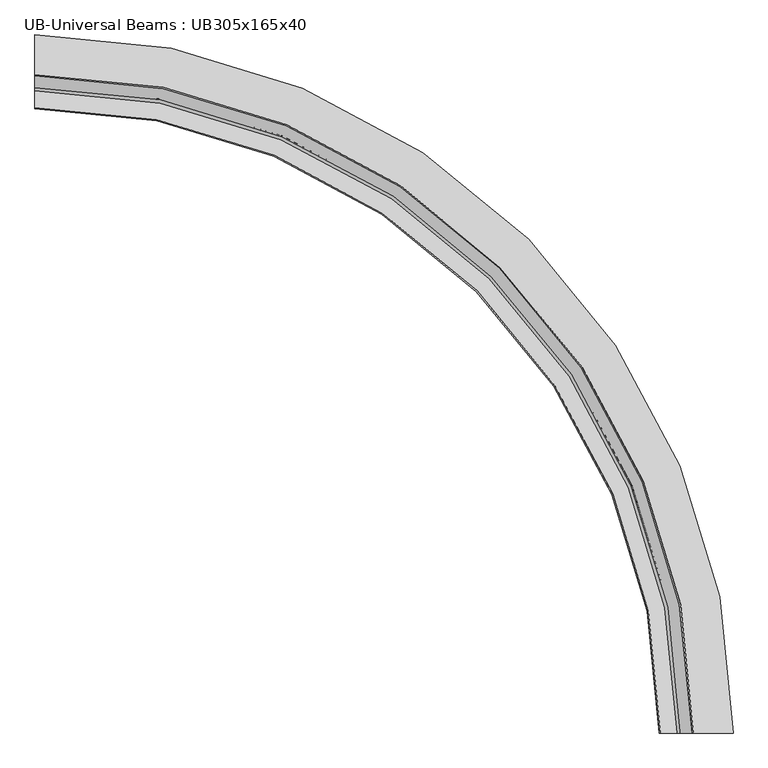
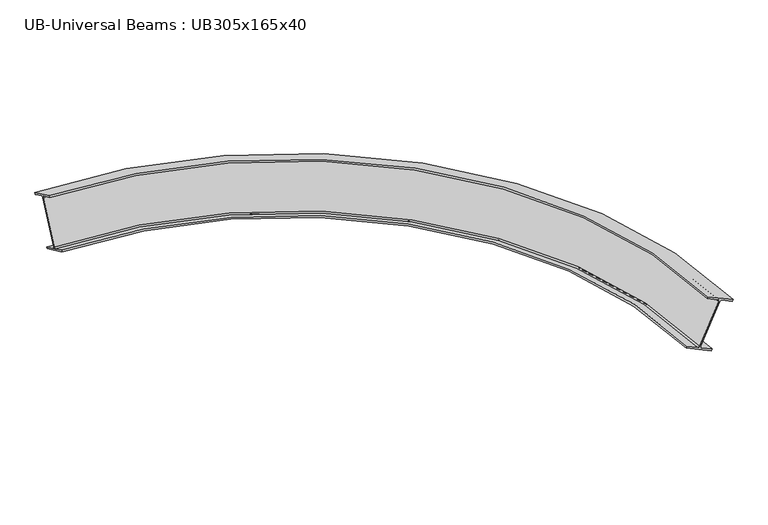
"""IFC4 building model written with IfcOpenShell, lengths in millimetres: beam geometry, UB-Universal Beams : UB305x165x40."""

from ifc_helpers import new_model, si_unit, point, frame, origin, place, context, project, spatial, polyline, circle_curve, ellipse_curve, trimmed, source, transform, mapped, element, save
from ifc_brep_helpers import plane_surface, revolved_surface, advanced_brep


def ub_universal_beams_ub305x165x40_80cf76f0(model_context):
    return source(origin(), model_context, "Body", "AdvancedBrep", [
        advanced_brep(
        [(2496.4431304, -2481.473222, -163.1085585), (2432.4578006, -2481.473222, -133.2717092), (2428.1529638, -2481.473222, -121.4442673), (2540.2313268, -2481.473222, 118.9085578), (2552.0587687, -2481.473222, 123.2133946), (2616.0440984, -2481.473222, 93.3765453), (2620.3548047, -2481.473222, 102.6208847), (2470.8140198, -2481.473222, 172.3528979), (2466.5033136, -2481.473222, 163.1085585), (2530.4886433, -2481.473222, 133.2717092), (2534.7934801, -2481.473222, 121.4442673), (2422.7151171, -2481.473222, -118.9085578), (2410.8876753, -2481.473222, -123.2133946), (2346.9023455, -2481.473222, -93.3765453), (2342.5916392, -2481.473222, -102.6208847), (2492.1324241, -2481.473222, -172.3528979), (0.0, 14.9699084, -163.1085585), (0.0, 10.6592021, -172.3528979), (0.0, -138.8815827, -102.6208847), (0.0, -134.5708765, -93.3765453), (0.0, -70.5855467, -123.2133946), (0.0, -58.7581049, -118.9085578), (0.0, 53.3202581, 121.4442673), (0.0, 49.0154214, 133.2717092), (0.0, -14.9699084, 163.1085585), (0.0, -10.6592021, 172.3528979), (0.0, 138.8815827, 102.6208847), (0.0, 134.5708765, 93.3765453), (0.0, 70.5855467, 123.2133946), (0.0, 58.7581049, 118.9085578), (0.0, -53.3202581, -121.4442673), (0.0, -49.0154214, -133.2717092)],
        [
            (0, 1),
            (1, 2, circle_curve(frame((2436.2191031, -2481.473222, -125.2055699), z_axis=(0.0, 1.0, 0.0), x_axis=(-0.9063077870366502, 0.0, 0.4226182617406989)), 8.9)),
            (2, 3),
            (3, 4, circle_curve(frame((2548.2974661, -2481.473222, 115.1472552), z_axis=(0.0, 1.0, 0.0), x_axis=(-0.9063077870366502, 0.0, 0.4226182617406989)), 8.9)),
            (4, 5),
            (5, 6),
            (6, 7),
            (7, 8),
            (8, 9),
            (9, 10, circle_curve(frame((2526.7273408, -2481.473222, 125.2055699), z_axis=(0.0, 1.0, 0.0), x_axis=(-0.9063077870366502, 0.0, 0.4226182617406989)), 8.9)),
            (10, 11),
            (11, 12, circle_curve(frame((2414.6489778, -2481.473222, -115.1472552), z_axis=(0.0, 1.0, 0.0), x_axis=(-0.9063077870366502, 0.0, 0.4226182617406989)), 8.9)),
            (12, 13),
            (13, 14),
            (14, 15),
            (15, 0),
            (16, 17),
            (17, 18),
            (18, 19),
            (19, 20),
            (20, 21, circle_curve(frame((0.0, -66.8242442, -115.1472552), z_axis=(1.0, 0.0, 0.0), x_axis=(0.0, -0.9063077870366502, 0.422618261740699)), 8.9)),
            (21, 22),
            (22, 23, circle_curve(frame((0.0, 45.2541188, 125.2055699), z_axis=(1.0, 0.0, 0.0), x_axis=(0.0, -0.9063077870366502, 0.422618261740699)), 8.9)),
            (23, 24),
            (24, 25),
            (25, 26),
            (26, 27),
            (27, 28),
            (28, 29, circle_curve(frame((0.0, 66.8242442, 115.1472552), z_axis=(1.0, 0.0, 0.0), x_axis=(0.0, -0.9063077870366502, 0.422618261740699)), 8.9)),
            (29, 30),
            (30, 31, circle_curve(frame((0.0, -45.2541188, -125.2055699), z_axis=(1.0, 0.0, 0.0), x_axis=(0.0, -0.9063077870366502, 0.422618261740699)), 8.9)),
            (31, 16),
            (0, 16, circle_curve(frame((0.0, -2481.473222, -163.1085585), z_axis=(0.0, 0.0, 1.0), x_axis=(0.0, 1.0, 0.0)), 2496.4431304)),
            (31, 1, circle_curve(frame((0.0, -2481.473222, -133.2717092), z_axis=(0.0, 0.0, -1.0), x_axis=(0.0, 1.0, 0.0)), 2432.4578006)),
            (30, 2, circle_curve(frame((0.0, -2481.473222, -121.4442673), z_axis=(0.0, 0.0, -1.0), x_axis=(0.0, 1.0, 0.0)), 2428.1529638)),
            (29, 3, circle_curve(frame((0.0, -2481.473222, 118.9085578), z_axis=(0.0, 0.0, -1.0), x_axis=(0.0, 1.0, 0.0)), 2540.2313268)),
            (28, 4, circle_curve(frame((0.0, -2481.473222, 123.2133946), z_axis=(0.0, 0.0, -1.0), x_axis=(0.0, 1.0, 0.0)), 2552.0587687)),
            (27, 5, circle_curve(frame((0.0, -2481.473222, 93.3765453), z_axis=(0.0, 0.0, -1.0), x_axis=(0.0, 1.0, 0.0)), 2616.0440984)),
            (26, 6, circle_curve(frame((0.0, -2481.473222, 102.6208847), z_axis=(0.0, 0.0, -1.0), x_axis=(0.0, 1.0, 0.0)), 2620.3548047)),
            (25, 7, circle_curve(frame((0.0, -2481.473222, 172.3528979), z_axis=(0.0, 0.0, -1.0), x_axis=(0.0, 1.0, 0.0)), 2470.8140198)),
            (24, 8, circle_curve(frame((0.0, -2481.473222, 163.1085585), z_axis=(0.0, 0.0, -1.0), x_axis=(0.0, 1.0, 0.0)), 2466.5033136)),
            (23, 9, circle_curve(frame((0.0, -2481.473222, 133.2717092), z_axis=(0.0, 0.0, -1.0), x_axis=(0.0, 1.0, 0.0)), 2530.4886433)),
            (22, 10, circle_curve(frame((0.0, -2481.473222, 121.4442673), z_axis=(0.0, 0.0, -1.0), x_axis=(0.0, 1.0, 0.0)), 2534.7934801)),
            (21, 11, circle_curve(frame((0.0, -2481.473222, -118.9085578), z_axis=(0.0, 0.0, -1.0), x_axis=(0.0, 1.0, 0.0)), 2422.7151171)),
            (20, 12, circle_curve(frame((0.0, -2481.473222, -123.2133946), z_axis=(0.0, 0.0, -1.0), x_axis=(0.0, 1.0, 0.0)), 2410.8876753)),
            (19, 13, circle_curve(frame((0.0, -2481.473222, -93.3765453), z_axis=(0.0, 0.0, -1.0), x_axis=(0.0, 1.0, 0.0)), 2346.9023455)),
            (18, 14, circle_curve(frame((0.0, -2481.473222, -102.6208847), z_axis=(0.0, 0.0, -1.0), x_axis=(0.0, 1.0, 0.0)), 2342.5916392)),
            (17, 15, circle_curve(frame((0.0, -2481.473222, -172.3528979), z_axis=(0.0, 0.0, -1.0), x_axis=(0.0, 1.0, 0.0)), 2492.1324241)),
        ],
        [
            plane_surface(frame((2481.473222, -2481.473222, 0.0), z_axis=(0.0, -1.0, 0.0), x_axis=(0.42261826174069883, 0.0, 0.9063077870366503))),
            plane_surface(frame((0.0, 0.0, 0.0), z_axis=(-1.0, 0.0, 0.0), x_axis=(0.0, 0.422618261740699, 0.9063077870366502))),
            revolved_surface(polyline([(0.0, -49.0154214, -133.2717092), (0.0, 14.9699084, -163.1085585)]), (0.0, -2481.473222, 0.0), (0.0, 0.0, -1.0)),
            revolved_surface(trimmed(ellipse_curve(frame((0.0, -45.2541188, -125.2055699), z_axis=(1.0, 0.0, 0.0), x_axis=(0.0, -0.9063077870366502, 0.422618261740699)), 8.9, 8.9), [point((0.0, -53.3202581, -121.4442673))], [point((0.0, -49.0154214, -133.2717092))], True, "CARTESIAN"), (0.0, -2481.473222, 0.0), (0.0, 0.0, -1.0)),
            revolved_surface(polyline([(0.0, 58.7581049, 118.9085578), (0.0, -53.3202581, -121.4442673)]), (0.0, -2481.473222, 0.0), (0.0, 0.0, -1.0)),
            revolved_surface(trimmed(ellipse_curve(frame((0.0, 66.8242442, 115.1472552), z_axis=(1.0, 0.0, 0.0), x_axis=(0.0, -0.9063077870366502, 0.422618261740699)), 8.9, 8.9), [point((0.0, 70.5855467, 123.2133946))], [point((0.0, 58.7581049, 118.9085578))], True, "CARTESIAN"), (0.0, -2481.473222, 0.0), (0.0, 0.0, -1.0)),
            revolved_surface(polyline([(0.0, 134.5708765, 93.3765453), (0.0, 70.5855467, 123.2133946)]), (0.0, -2481.473222, 0.0), (0.0, 0.0, -1.0)),
            revolved_surface(polyline([(0.0, 138.8815827, 102.6208847), (0.0, 134.5708765, 93.3765453)]), (0.0, -2481.473222, 0.0), (0.0, 0.0, -1.0)),
            revolved_surface(polyline([(0.0, -10.6592021, 172.3528979), (0.0, 138.8815827, 102.6208847)]), (0.0, -2481.473222, 0.0), (0.0, 0.0, -1.0)),
            revolved_surface(polyline([(0.0, -14.9699084, 163.1085585), (0.0, -10.6592021, 172.3528979)]), (0.0, -2481.473222, 0.0), (0.0, 0.0, -1.0)),
            revolved_surface(polyline([(0.0, 49.0154214, 133.2717092), (0.0, -14.9699084, 163.1085585)]), (0.0, -2481.473222, 0.0), (0.0, 0.0, -1.0)),
            revolved_surface(trimmed(ellipse_curve(frame((0.0, 45.2541188, 125.2055699), z_axis=(1.0, 0.0, 0.0), x_axis=(0.0, -0.9063077870366502, 0.422618261740699)), 8.9, 8.9), [point((0.0, 53.3202581, 121.4442673))], [point((0.0, 49.0154214, 133.2717092))], True, "CARTESIAN"), (0.0, -2481.473222, 0.0), (0.0, 0.0, -1.0)),
            revolved_surface(polyline([(0.0, -58.7581049, -118.9085578), (0.0, 53.3202581, 121.4442673)]), (0.0, -2481.473222, 0.0), (0.0, 0.0, -1.0)),
            revolved_surface(trimmed(ellipse_curve(frame((0.0, -66.8242442, -115.1472552), z_axis=(1.0, 0.0, 0.0), x_axis=(0.0, -0.9063077870366502, 0.422618261740699)), 8.9, 8.9), [point((0.0, -70.5855467, -123.2133946))], [point((0.0, -58.7581049, -118.9085578))], True, "CARTESIAN"), (0.0, -2481.473222, 0.0), (0.0, 0.0, -1.0)),
            revolved_surface(polyline([(0.0, -134.5708765, -93.3765453), (0.0, -70.5855467, -123.2133946)]), (0.0, -2481.473222, 0.0), (0.0, 0.0, -1.0)),
            revolved_surface(polyline([(0.0, -138.8815827, -102.6208847), (0.0, -134.5708765, -93.3765453)]), (0.0, -2481.473222, 0.0), (0.0, 0.0, -1.0)),
            revolved_surface(polyline([(0.0, 10.6592021, -172.3528979), (0.0, -138.8815827, -102.6208847)]), (0.0, -2481.473222, 0.0), (0.0, 0.0, -1.0)),
            revolved_surface(polyline([(0.0, 14.9699084, -163.1085585), (0.0, 10.6592021, -172.3528979)]), (0.0, -2481.473222, 0.0), (0.0, 0.0, -1.0)),
        ],
        [
            (0, [[1, 2, 3, 4, 5, 6, 7, 8, 9, 10, 11, 12, 13, 14, 15, 16]]),
            (1, [[17, 18, 19, 20, 21, 22, 23, 24, 25, 26, 27, 28, 29, 30, 31, 32]]),
            (2, [[-1, 33, -32, 34]]),
            (3, [[-2, -34, -31, 35]]),
            (4, [[-3, -35, -30, 36]]),
            (5, [[-4, -36, -29, 37]]),
            (6, [[-5, -37, -28, 38]]),
            (7, [[-6, -38, -27, 39]]),
            (8, [[-7, -39, -26, 40]]),
            (9, [[-8, -40, -25, 41]]),
            (10, [[-9, -41, -24, 42]]),
            (11, [[-10, -42, -23, 43]]),
            (12, [[-11, -43, -22, 44]]),
            (13, [[-12, -44, -21, 45]]),
            (14, [[-13, -45, -20, 46]]),
            (15, [[-14, -46, -19, 47]]),
            (16, [[-15, -47, -18, 48]]),
            (17, [[-16, -48, -17, -33]]),
        ],
    ),
    ])


if __name__ == "__main__":
    model = new_model("IFC4")
    model_context = context("Model", 3, world=origin())
    ifc_project = project(units=[si_unit("LENGTHUNIT", "METRE", prefix="MILLI")], contexts=[model_context])
    site = spatial("IfcSite", under=ifc_project)
    building = spatial("IfcBuilding", under=site)
    placement = place(None, origin())
    ub_universal_beams_ub305x165x40_shape = ub_universal_beams_ub305x165x40_80cf76f0(model_context)
    element("IfcBeam", 1, ObjectType="UB-Universal Beams : UB305x165x40", at=placement, inside=building, context=model_context, shape_type="MappedRepresentation", body=[
        mapped(ub_universal_beams_ub305x165x40_shape, transform((0.0, 0.0, 0.0), x_axis=(1.0, 0.0, 0.0), y_axis=(0.0, 1.0, 0.0), z_axis=(0.0, 0.0, 1.0))),
    ])
    save(model, "model.ifc")

# Revit data of these elements
# Type "UB-Universal Beams : UB305x165x40"
#   Section Name Key = "UB305X165X40"
#   Width = 16.5 cm
#   Web Thickness = 0.6 cm
#   Web Fillet = 0.89 cm
#   Warping Constant = 164000.0 cm⁶
#   Torsional Moment of Inertia = 14.70 cm⁴
#   Section Area = 51.3 cm²
#   Plastic Modulus weak axis = 142.0 cm³
#   Plastic Modulus strong axis = 623.0 cm³
#   Nominal Weight = 40.2999 kgf/m
#   Moment of Inertia weak axis = 764.00 cm⁴
#   Moment of Inertia strong axis = 8503.00 cm⁴
#   Height = 30.34 cm
#   Flange Thickness = 1.02 cm
#   Elastic Modulus weak axis = 92.6 cm³
#   Elastic Modulus strong axis = 560.0 cm³
#   Centroid Vertical = 15.17 cm
#   Centroid Horizontal = 8.25 cm
#   Bolt Spacing = 9.0 cm
#   Length [instance default] = 1500 mm
#   Structural Material [instance default] = Metal - Steel 43-275
#   Type Comments = ""
#   Assembly Code = ""
# Element 1 (IfcBeam, "UB-Universal Beams : UB305x165x40")
#   Materials on its faces: "Metal - Steel 43-275"
# Materials
#   "Metal - Steel 43-275": class "Metal", colour RGB 247 247 247, transparency 0, Cost = 0
